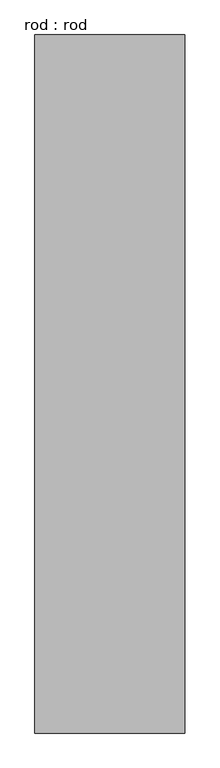
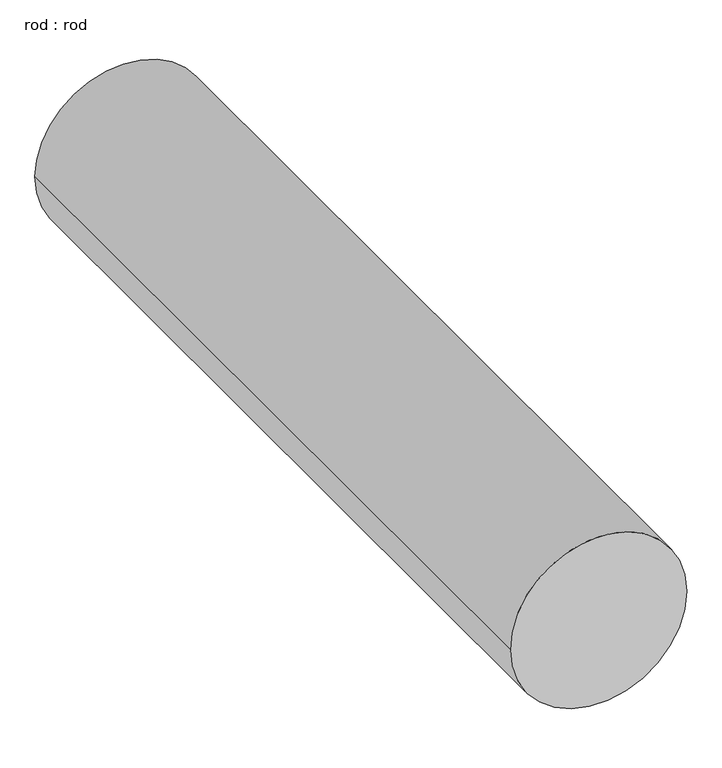
"""IFC4 building model written with IfcOpenShell, lengths in millimetres: proxy geometry, rod : rod."""

from ifc_helpers import new_model, si_unit, point, frame, frame_2d, origin, place, context, project, spatial, circle_curve, trimmed, segment, composite_curve, outline, extrude, source, transform, mapped, element, save


def rod_rod_412d9cae(model_context):
    return source(origin(), model_context, "Body", "SweptSolid", [
        extrude(outline(composite_curve([segment(trimmed(circle_curve(frame_2d((0.0108462, 0.0)), 200.0), [point((0.0108462, 200.0))], [point((0.0108462, -200.0))], False, "CARTESIAN"), True, "CONTINUOUS"), segment(trimmed(circle_curve(frame_2d((0.0108462, 0.0)), 200.0), [point((0.0108462, -200.0))], [point((0.0108462, 200.0))], False, "CARTESIAN"), True, "CONTINUOUS")], self_intersect=False)), frame((0.0, 3159.9807744, 0.0), z_axis=(0.0, 1.0, 0.0), x_axis=(0.0, 0.0, 1.0)), (0.0, 0.0, 1.0), 1865.4956819),
    ])


if __name__ == "__main__":
    model = new_model("IFC4")
    model_context = context("Model", 3, world=origin())
    ifc_project = project(units=[si_unit("LENGTHUNIT", "METRE", prefix="MILLI")], contexts=[model_context])
    site = spatial("IfcSite", under=ifc_project)
    building = spatial("IfcBuilding", under=site)
    placement = place(None, origin())
    rod_rod_shape = rod_rod_412d9cae(model_context)
    element("IfcBuildingElementProxy", 1, Name="rod : rod", ObjectType="rod : rod", at=placement, inside=building, context=model_context, shape_type="MappedRepresentation", body=[
        mapped(rod_rod_shape, transform((0.0, 0.0, 0.0), x_axis=(1.0, 0.0, 0.0), y_axis=(0.0, 1.0, 0.0), z_axis=(0.0, 0.0, 1.0))),
    ])
    save(model, "model.ifc")

# Revit data of these elements
# Type "rod : rod"
#   Default Elevation = 0
